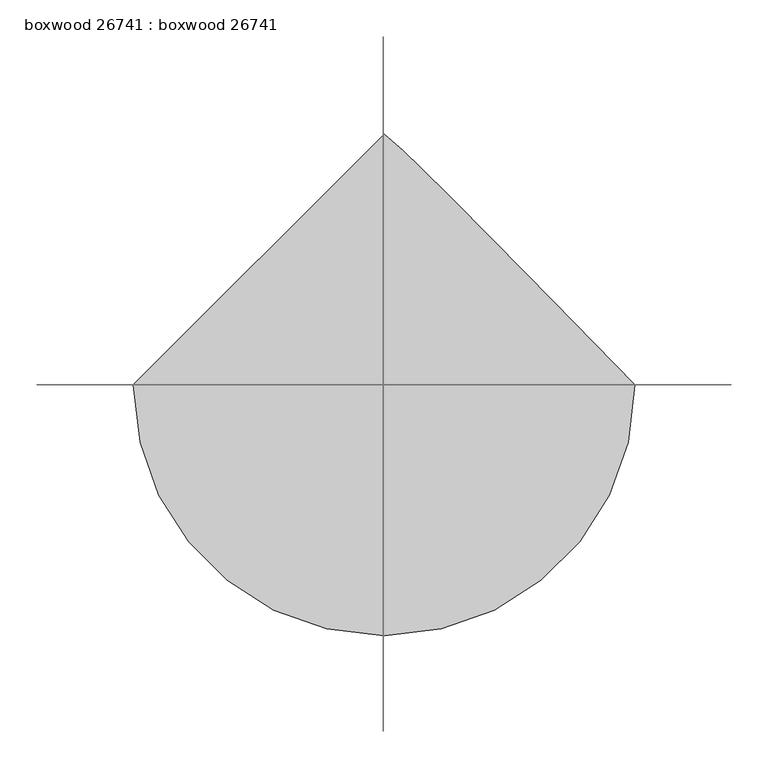
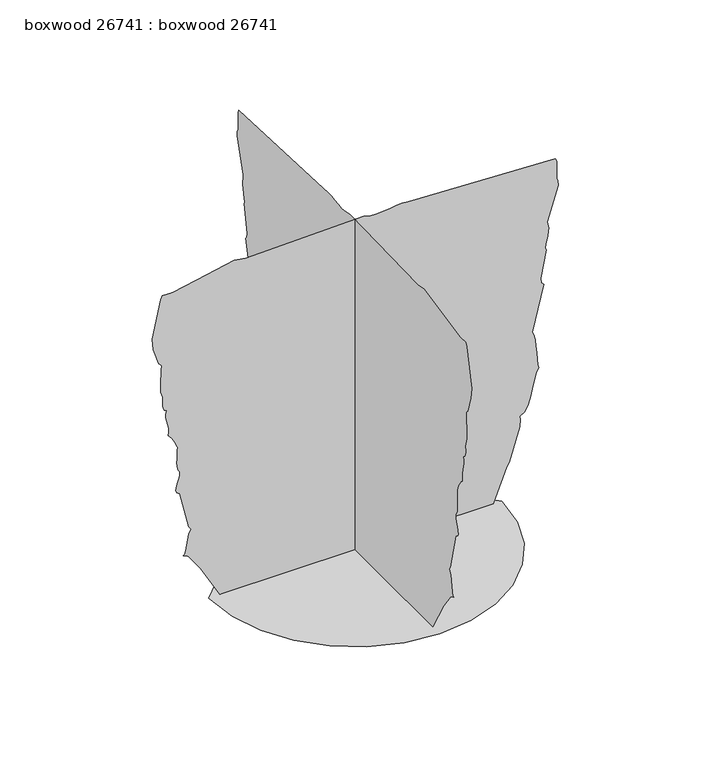
"""IFC4 building model written with IfcOpenShell, lengths in millimetres: proxy geometry, boxwood 26741 : boxwood 26741."""

import ifcopenshell
import ifcopenshell.guid

model = None  # the IFC model being written
_history = None  # IfcOwnerHistory: only IFC2X3 demands one
_inside = {}  # id of a spatial element -> (the spatial element, [elements in it])
_under = {}  # id of a project, library or spatial element -> (it, [spatial elements below it])
_declared = {}  # id of a project -> (the project, [libraries it declares])
_typed = {}  # id of a type object -> (the type object, [elements of that type])
_made_of = {}  # id of a material, layer set ... -> (it, [elements and type objects made of it])


def new_model(schema):
    """Start an empty IFC model of exactly this schema.

    Asked for "IFC4X3", IfcOpenShell would pick the latest addendum, in which some entities
    have other attributes; the version numbers below select the first issue.
    IFC2X3 requires an IfcOwnerHistory on every rooted entity: one is made here for all.
    """
    global model, _history
    if schema == "IFC4X3":
        model = ifcopenshell.file(schema_version=(4, 3, 0, 0))
    else:
        model = ifcopenshell.file(schema=schema)
    _inside.clear()
    _under.clear()
    _declared.clear()
    _typed.clear()
    _made_of.clear()
    _history = None
    if model.schema == "IFC2X3":
        org = make("IfcOrganization", Name="unknown")
        user = make(
            "IfcPersonAndOrganization",
            ThePerson=make("IfcPerson", FamilyName="unknown"),
            TheOrganization=org,
        )
        app = make(
            "IfcApplication",
            ApplicationDeveloper=org,
            Version="unknown",
            ApplicationFullName="unknown",
            ApplicationIdentifier="unknown",
        )
        _history = make(
            "IfcOwnerHistory",
            OwningUser=user,
            OwningApplication=app,
            ChangeAction="ADDED",
            CreationDate=0,
        )
    return model


def make(cls, **values):
    """One entity of the class cls with the attributes given. An attribute that is None is left unset."""
    return model.create_entity(
        cls, **{name: value for name, value in values.items() if value is not None}
    )


def rooted(cls, **values):
    """An entity with a GlobalId (a new one), such as an element, a storey or a relation."""
    return make(cls, GlobalId=ifcopenshell.guid.new(), OwnerHistory=_history, **values)


def si_unit(unit_type, name, prefix=None):
    """IfcSIUnit, for example si_unit("LENGTHUNIT", "METRE", prefix="MILLI")."""
    return make("IfcSIUnit", UnitType=unit_type, Prefix=prefix, Name=name)


def assignment(units):
    """IfcUnitAssignment: the units of a project."""
    return None if units is None else make("IfcUnitAssignment", Units=units)


def point(xyz):
    """IfcCartesianPoint."""
    return None if xyz is None else make("IfcCartesianPoint", Coordinates=xyz)


def direction(xyz):
    """IfcDirection."""
    return None if xyz is None else make("IfcDirection", DirectionRatios=xyz)


def frame(location, z_axis=None, x_axis=None):
    """IfcAxis2Placement3D, a coordinate frame: its origin and axes. An axis left out is left unset."""
    return make(
        "IfcAxis2Placement3D",
        Location=point(location),
        Axis=direction(z_axis),
        RefDirection=direction(x_axis),
    )


def origin():
    """The frame at (0, 0, 0) with its axes left unset."""
    return frame((0.0, 0.0, 0.0))


def place(relative_to, where):
    """IfcLocalPlacement: puts the frame where relative to a parent placement (None: the world)."""
    return make(
        "IfcLocalPlacement", PlacementRelTo=relative_to, RelativePlacement=where
    )


def context(
    kind, dimensions, precision=None, world=None, true_north=None, identifier=None
):
    """IfcGeometricRepresentationContext, for example the 3D "Model" context."""
    return make(
        "IfcGeometricRepresentationContext",
        ContextIdentifier=identifier,
        ContextType=kind,
        CoordinateSpaceDimension=dimensions,
        Precision=precision,
        WorldCoordinateSystem=world,
        TrueNorth=true_north,
    )


def project(units=None, contexts=None):
    """IfcProject with its units and contexts."""
    return rooted(
        "IfcProject",
        Name="project",
        RepresentationContexts=contexts,
        UnitsInContext=assignment(units),
    )


def spatial(cls, under=None, at=None, **own):
    """A site, building, storey or space (cls), placed at a placement, below another one or the project."""
    s = rooted(cls, ObjectPlacement=at, **own)
    if under is not None:
        _under.setdefault(under.id(), (under, []))[1].append(s)
    return s


def point_list(points):
    """IfcCartesianPointList2D or 3D."""
    cls = (
        "IfcCartesianPointList2D" if len(points[0]) == 2 else "IfcCartesianPointList3D"
    )
    return make(cls, CoordList=points)


def triangles(points, corners, closed=None, point_numbers=None):
    """IfcTriangulatedFaceSet: each triangle names its three corners, points numbered from 1."""
    return make(
        "IfcTriangulatedFaceSet",
        Coordinates=point_list(points),
        Closed=closed,
        CoordIndex=corners,
        PnIndex=point_numbers,
    )


def shape(context_of_items, identifier, shape_type, items):
    """IfcShapeRepresentation: the items that make up one representation, for example the "Body"."""
    return make(
        "IfcShapeRepresentation",
        ContextOfItems=context_of_items,
        RepresentationIdentifier=identifier,
        RepresentationType=shape_type,
        Items=items,
    )


def source(mapping_origin, context_of_items, identifier, shape_type, items):
    """IfcRepresentationMap: a shape defined once, which mapped items show again and again."""
    return make(
        "IfcRepresentationMap",
        MappingOrigin=mapping_origin,
        MappedRepresentation=shape(context_of_items, identifier, shape_type, items),
    )


def transform(
    local_origin,
    x_axis=None,
    y_axis=None,
    z_axis=None,
    scale=None,
    scale2=None,
    scale3=None,
    uniform=True,
):
    """IfcCartesianTransformationOperator3D, or its non-uniform kind. x_axis, y_axis, z_axis: its Axis1, 2, 3."""
    if uniform:
        return make(
            "IfcCartesianTransformationOperator3D",
            Axis1=direction(x_axis),
            Axis2=direction(y_axis),
            LocalOrigin=point(local_origin),
            Scale=scale,
            Axis3=direction(z_axis),
        )
    return make(
        "IfcCartesianTransformationOperator3DnonUniform",
        Axis1=direction(x_axis),
        Axis2=direction(y_axis),
        LocalOrigin=point(local_origin),
        Scale=scale,
        Axis3=direction(z_axis),
        Scale2=scale2,
        Scale3=scale3,
    )


def mapped(mapping_source, mapping_target):
    """IfcMappedItem: shows the shape of a source again, moved by a transform."""
    return make(
        "IfcMappedItem", MappingSource=mapping_source, MappingTarget=mapping_target
    )


def made_of(thing, what):
    """Note that an element or type object is made of a material, layer set ...; save() writes the relation."""
    if what is not None:
        _made_of.setdefault(what.id(), (what, []))[1].append(thing)
    return thing


def element(
    cls,
    number,
    at=None,
    inside=None,
    cuts=None,
    type_object=None,
    material=None,
    context=None,
    identifier="Body",
    shape_type=None,
    held_by="IfcProductDefinitionShape",
    body=None,
    shapes=None,
    **own,
):
    """One element of the class cls, such as IfcWall. Its Tag is "e" and its number.

    at: its placement. inside: the storey or other place that contains it. cuts: it is an
    opening in that element (IfcRelVoidsElement). A single representation is given by context,
    identifier, shape_type and body (its items); several are given by shapes. held_by: the class
    of the entity that holds the representations. save() writes the other relations.
    """
    e = rooted(cls, Tag="e%d" % number, ObjectPlacement=at, **own)
    if body is not None:
        shapes = [shape(context, identifier, shape_type, body)]
    if shapes is not None:
        e.Representation = make(held_by, Representations=shapes)
    if inside is not None:
        _inside.setdefault(inside.id(), (inside, []))[1].append(e)
    if cuts is not None:
        rooted(
            "IfcRelVoidsElement", RelatingBuildingElement=cuts, RelatedOpeningElement=e
        )
    if type_object is not None:
        _typed.setdefault(type_object.id(), (type_object, []))[1].append(e)
    return made_of(e, material)


def aggregate(whole, parts):
    """IfcRelAggregates: a whole, such as a stair, and the parts it consists of."""
    return rooted("IfcRelAggregates", RelatingObject=whole, RelatedObjects=parts)


def save(model, path):
    """Write the relations noted so far, then the file.

    IfcRelAggregates (storeys below a building ...), IfcRelContainedInSpatialStructure (elements
    in a storey), IfcRelDefinesByType, IfcRelAssociatesMaterial and IfcRelDeclares: one each for
    every whole, place, type object, material and project.
    """
    for whole, parts in _under.values():
        aggregate(whole, parts)
    for where, things in _inside.values():
        rooted(
            "IfcRelContainedInSpatialStructure",
            RelatedElements=things,
            RelatingStructure=where,
        )
    for kind, things in _typed.values():
        rooted("IfcRelDefinesByType", RelatedObjects=things, RelatingType=kind)
    for what, things in _made_of.values():
        rooted("IfcRelAssociatesMaterial", RelatedObjects=things, RelatingMaterial=what)
    for by, libraries in _declared.values():
        rooted("IfcRelDeclares", RelatingContext=by, RelatedDefinitions=libraries)
    model.write(path)


def boxwood_26741_boxwood_26741_9aa5a226(model_context):
    return source(origin(), model_context, "Body", "Tessellation", [
        triangles([(-340.161904, 0.0, 0.0), (-331.1677583, -77.9424445, 0.0), (-305.5569305, -149.5201522, 0.0), (-265.3792049, -212.6823306, 0.0), (-212.6823306, -265.3792049, 0.0), (-149.5201522, -305.5569305, 0.0), (-77.9424445, -331.1677583, 0.0), (1.49e-05, -340.161904, 0.0), (77.9424445, -331.1677583, 0.0), (149.5201522, -305.5569305, 0.0), (212.6823306, -265.3792049, 0.0), (265.3792049, -212.6823306, 0.0), (305.5569305, -149.5201522, 0.0), (331.1677583, -77.9424445, 0.0), (340.161904, 2.97e-05, 0.0), (229.6165077, 113.3919522, 0.0), (147.6639246, 196.877445, 0.0), (89.5385572, 255.4401858, 0.0), (50.4748806, 294.0659713, 0.0), (25.7075946, 317.7387815, 0.0), (10.4710485, 331.4420875, 0.0), (-4.46e-05, 340.161904, 0.0), (-314.391057, 3.72e-05, 1.1804295), (-359.6030502, 3.25e-05, 80.9365932), (-387.8072153, 3.02e-05, 119.3439327), (-399.7375917, 2.98e-05, 125.1409807), (-396.5295753, 2.97e-05, 127.6759005), (-393.8092472, 2.92e-05, 136.0634881), (-391.3784363, 2.85e-05, 147.9626255), (-389.0442038, 2.77e-05, 161.0321948), (-386.6159363, 2.7e-05, 172.9315956), (-383.8930647, 2.65e-05, 181.3191832), (-380.6875917, 2.64e-05, 183.8540939), (-386.4178379, 2.59e-05, 191.475867), (-407.8706709, 2.06e-05, 279.9816748), (-415.0715758, 2.03e-05, 285.8922515), (-417.4159822, 1.99e-05, 291.1246538), (-416.3669546, 1.95e-05, 298.5846272), (-413.3773842, 1.9e-05, 307.4187355), (-409.9052124, 1.84e-05, 316.7735787), (-407.3982433, 1.79e-05, 325.7905792), (-407.3144185, 1.74e-05, 333.6213876), (-411.0989985, 1.7e-05, 339.4049735), (-412.8821019, 1.68e-05, 343.3826014), (-413.8320439, 1.64e-05, 350.1263031), (-414.1444885, 1.59e-05, 358.7927799), (-414.0123745, 1.54e-05, 368.5362259), (-413.6237718, 1.48e-05, 378.5158856), (-413.1741989, 1.42e-05, 387.8859532), (-412.8516169, 1.37e-05, 395.8056733), (-413.5475773, 1.36e-05, 397.7894185), (-415.5668581, 1.33e-05, 402.5595489), (-418.5996308, 1.29e-05, 409.0720874), (-422.335958, 1.25e-05, 416.2857096), (-426.4660111, 1.21e-05, 423.1538587), (-430.6849397, 1.17e-05, 428.6300869), (-434.6803717, 1.15e-05, 431.6729971), (-433.0471501, 1.1e-05, 440.9821309), (-433.7685087, 1.04e-05, 450.5350362), (-435.8335353, 9.9e-06, 460.1032385), (-438.2363683, 9.3e-06, 469.4580454), (-439.9737259, 8.8e-06, 478.3709098), (-440.034696, 8.3e-06, 486.6106685), (-437.4134171, 7.8e-06, 493.9512815), (-443.2020899, 7.6e-06, 497.9797056), (-446.1205164, 7.3e-06, 503.1613297), (-447.0831757, 6.9e-06, 509.2624108), (-447.0095246, 6.6e-06, 516.0543654), (-446.8114263, 6.1e-06, 523.3111536), (-447.4083012, 5.6e-06, 530.7990686), (-449.7146284, 5.2e-06, 538.2920706), (-451.312278, 4.9e-06, 544.3448625), (-452.0082384, 4.4e-06, 552.960543), (-452.0184122, 3.7e-06, 563.4380648), (-451.5713828, 3e-06, 575.0738008), (-450.8830164, 2.3e-06, 587.161653), (-450.1769185, 1.6e-06, 599.0006106), (-449.6740059, 1e-06, 609.884503), (-455.9351063, 5e-07, 616.20403), (-468.9576762, -1.9e-06, 655.9295849), (-471.3528789, -3.4e-06, 681.38806), (-452.1758881, -8.8e-06, 772.6680262), (-448.2312887, -9.3e-06, 780.8340975), (-424.9242448, -9.2e-06, 779.2695127), (-369.5370006, -9.9e-06, 791.4970367), (-280.9036933, -1.1e-05, 809.3710184), (-254.2463815, -1.07e-05, 804.8396816), (19.1367407, -1.11e-05, 811.6748022), (35.370009, -1.09e-05, 807.659059), (50.7118619, -1.08e-05, 806.6938562), (65.4184633, -1.09e-05, 807.7555647), (79.7468584, -1.1e-05, 809.8129972), (93.9523139, -1.11e-05, 811.837365), (108.2921454, -1.11e-05, 812.8000242), (123.0221057, -1.11e-05, 811.6748022), (464.7514286, -1.02e-05, 797.3212452), (467.4463586, -9.9e-06, 790.6791361), (467.5250965, -7.3e-06, 748.7767519), (470.2200628, -6.9e-06, 742.132172), (471.0074421, -6.3e-06, 730.722476), (446.1992907, -1.4e-06, 649.650753), (447.5784943, -8e-07, 638.6728621), (448.9932698, -4e-07, 632.8486536), (448.3227076, 0.0, 624.6114384), (446.3999325, 6e-07, 614.9264191), (444.0605767, 1.2e-06, 604.756255), (442.1378016, 1.8e-06, 595.0686922), (441.4672394, 2.3e-06, 586.8314406), (442.8795078, 2.7e-06, 581.0072322), (430.5681227, 6.5e-06, 516.2728114), (432.2445102, 7.2e-06, 504.59896), (437.7537669, 7.6e-06, 498.820461), (410.7154827, 1.41e-05, 389.8950966), (414.6016554, 1.45e-05, 382.811045), (417.3397877, 1.52e-05, 370.1135642), (419.2981347, 1.62e-05, 353.9591723), (420.8348505, 1.72e-05, 336.5119088), (422.3156467, 1.82e-05, 319.9231685), (424.1038007, 1.9e-05, 306.3570271), (426.5625169, 1.95e-05, 297.9699481), (420.4843268, 2.02e-05, 287.3705225), (415.6710305, 2.11e-05, 270.9595874), (411.3047636, 2.23e-05, 251.374918), (406.5625749, 2.35e-05, 231.2497293), (400.6266, 2.46e-05, 213.2215782), (392.6738514, 2.54e-05, 199.9259508), (381.8813779, 2.58e-05, 193.9993685), (383.6035111, 2.63e-05, 184.6265031), (381.7493002, 2.73e-05, 168.2889829), (357.4541988, 3.19e-05, 89.6124717), (351.8814649, 3.25e-05, 80.6919951), (319.8571115, 3.72e-05, 1.0471049), (-1.3669569, -313.0245343, 1.1804269), (-1.3669569, -358.2365275, 80.9365932), (-1.3669569, -386.4381492, 119.3439327), (-1.3669569, -398.371069, 125.1409807), (-1.3669569, -395.1630527, 127.6759005), (-1.3669569, -392.4427245, 136.0634881), (-1.3669569, -390.0119136, 147.9626255), (-1.3669569, -387.6776811, 161.0324491), (-1.3669569, -385.2469065, 172.9315956), (-1.3669569, -382.526542, 181.3191832), (-1.3669569, -379.3185256, 183.8540939), (-1.3669569, -385.0513152, 191.475867), (-1.3669569, -406.5041482, 279.9816748), (-1.3669569, -413.7050531, 285.8922515), (-1.3669569, -416.046916, 291.1246538), (-1.3669569, -414.9979248, 298.5846272), (-1.3669569, -412.0108615, 307.4187355), (-1.3669569, -408.5386897, 316.7735787), (-1.3669569, -406.0317206, 325.7905792), (-1.3669569, -405.9453524, 333.6213876), (-1.3669569, -409.7324759, 339.4049735), (-1.3669569, -411.5130358, 343.3826014), (-1.3669569, -412.4655212, 350.1263031), (-1.3669569, -412.7779658, 358.7927799), (-1.3669569, -412.6458881, 368.5362259), (-1.3669569, -412.2572491, 378.5158856), (-1.3669569, -411.8076762, 387.8859532), (-1.3669569, -411.4850942, 395.8056733), (-1.3669569, -412.1810546, 397.7894185), (-1.3669569, -414.2003354, 402.5595489), (-1.3669569, -417.2331081, 409.0720874), (-1.3669569, -420.9669282, 416.2857096), (-1.3669569, -425.0994884, 423.1538587), (-1.3669569, -429.318417, 428.6300869), (-1.3669569, -433.3113055, 431.6729971), (-1.3669569, -431.6806274, 440.9821309), (-1.3669569, -432.401986, 450.5350362), (-1.3669569, -434.4670126, 460.1032385), (-1.3669569, -436.8698456, 469.4580454), (-1.3669569, -438.6046597, 478.3709098), (-1.3669569, -438.6681733, 486.6132119), (-1.3669569, -436.0468944, 493.9512815), (-1.3669569, -441.8355672, 497.9797056), (-1.3669569, -444.75403, 503.1613297), (-1.3669569, -445.7166893, 509.2624108), (-1.3669569, -445.6430019, 516.0543654), (-1.3669569, -445.4449036, 523.3111536), (-1.3669569, -446.0417785, 530.7990686), (-1.3669569, -448.3481057, 538.2920706), (-1.3669569, -449.9457553, 544.3448625), (-1.3669569, -450.6392086, 552.960543), (-1.3669569, -450.6518895, 563.4380648), (-1.3669569, -450.2023167, 575.0738008), (-1.3669569, -449.5139866, 587.161653), (-1.3669569, -448.8078524, 599.0006106), (-1.3669569, -448.3049397, 609.884503), (-1.3669569, -454.5685836, 616.20403), (-1.3669569, -467.5911535, 655.9295849), (-1.3669569, -469.9863562, 681.38806), (-1.3669569, -450.8093654, 772.6680262), (-1.3669569, -446.864766, 780.8340975), (-1.3669569, -423.5577221, 779.2695127), (-1.3669569, -368.1704779, 791.4970367), (-1.3669569, -279.5371706, 809.3710184), (-1.3669569, -252.8793683, 804.8396816), (-1.3669569, 20.5037698, 811.6748022), (-1.3669569, 36.7367838, 807.659059), (-1.3669569, 52.0788933, 806.6938562), (-1.3669569, 66.7854902, 807.7555647), (-1.3669569, 81.1138897, 809.8129972), (-1.3669569, 95.3193453, 811.837365), (-1.3669569, 109.6591677, 812.8000242), (-1.3669569, 124.3891371, 811.6748022), (-1.3669569, 466.1179513, 797.3212452), (-1.3669569, 468.8128813, 790.6791361), (-1.3669569, 468.8916192, 748.7767519), (-1.3669569, 471.5865855, 742.132172), (-1.3669569, 472.3739648, 730.722476), (-1.3669569, 447.565777, 649.650753), (-1.3669569, 448.9475604, 638.6754055), (-1.3669569, 450.3597925, 632.8486536), (-1.3669569, 449.6892303, 624.6114384), (-1.3669569, 447.7664552, 614.9264191), (-1.3669569, 445.4270994, 604.756255), (-1.3669569, 443.5068678, 595.0686922), (-1.3669569, 442.8337621, 586.8314406), (-1.3669569, 444.2485376, 581.0072322), (-1.3669569, 431.9371888, 516.2728114), (-1.3669569, 433.6135763, 504.59896), (-1.3669569, 439.1228331, 498.820461), (-1.3669569, 412.0820054, 389.8950966), (-1.3669569, 415.9681781, 382.811045), (-1.3669569, 418.7088538, 370.1135642), (-1.3669569, 420.6646574, 353.9591723), (-1.3669569, 422.2013369, 336.5119088), (-1.3669569, 423.6821694, 319.9231685), (-1.3669569, 425.4703234, 306.3570271), (-1.3669569, 427.9290396, 297.9699481), (-1.3669569, 421.8508495, 287.3705225), (-1.3669569, 417.0375169, 270.9595874), (-1.3669569, 412.6712863, 251.374918), (-1.3669569, 407.9290976, 231.2497293), (-1.3669569, 401.9931227, 213.2215782), (-1.3669569, 394.0403741, 199.9259508), (-1.3669569, 383.2479006, 193.9993685), (-1.3669569, 384.9700338, 184.6265031), (-1.3669569, 383.1158229, 168.2892373), (-1.3669569, 358.8207215, 89.6124717), (-1.3669569, 353.2479876, 80.6919951), (-1.3669569, 321.2261776, 1.0470998)], [[21, 22, 1], [20, 21, 1], [19, 20, 1], [18, 19, 1], [17, 18, 1], [17, 1, 2], [17, 2, 3], [17, 3, 4], [16, 17, 4], [16, 4, 5], [16, 5, 6], [16, 6, 7], [16, 7, 8], [16, 8, 9], [16, 9, 10], [16, 10, 11], [16, 11, 12], [15, 16, 12], [14, 15, 12], [13, 14, 12], [25, 26, 27], [131, 132, 23], [82, 83, 84], [95, 96, 97], [95, 97, 98], [25, 27, 28], [56, 57, 58], [131, 23, 24], [130, 131, 24], [129, 130, 24], [128, 129, 24], [127, 128, 24], [95, 98, 99], [95, 99, 100], [95, 100, 101], [95, 101, 102], [127, 24, 25], [127, 25, 28], [127, 28, 29], [127, 29, 30], [127, 30, 31], [127, 31, 32], [127, 32, 33], [127, 33, 34], [127, 34, 35], [111, 112, 113], [95, 102, 103], [95, 103, 104], [95, 104, 105], [95, 105, 106], [95, 106, 107], [95, 107, 108], [119, 120, 121], [81, 82, 84], [95, 108, 109], [95, 109, 110], [94, 95, 110], [93, 94, 110], [92, 93, 110], [91, 92, 110], [91, 110, 111], [90, 91, 111], [90, 111, 113], [89, 90, 113], [126, 127, 35], [125, 126, 35], [124, 125, 35], [123, 124, 35], [122, 123, 35], [121, 122, 35], [119, 121, 35], [118, 119, 35], [117, 118, 35], [116, 117, 35], [115, 116, 35], [114, 115, 35], [113, 114, 35], [89, 113, 35], [88, 89, 35], [87, 88, 35], [87, 35, 36], [87, 36, 37], [81, 84, 85], [80, 81, 85], [79, 80, 85], [78, 79, 85], [78, 85, 86], [78, 86, 87], [77, 78, 87], [76, 77, 87], [75, 76, 87], [74, 75, 87], [73, 74, 87], [72, 73, 87], [71, 72, 87], [70, 71, 87], [69, 70, 87], [68, 69, 87], [67, 68, 87], [66, 67, 87], [65, 66, 87], [64, 65, 87], [55, 56, 58], [62, 63, 64], [62, 64, 87], [61, 62, 87], [60, 61, 87], [59, 60, 87], [58, 59, 87], [55, 58, 87], [54, 55, 87], [53, 54, 87], [52, 53, 87], [51, 52, 87], [50, 51, 87], [49, 50, 87], [48, 49, 87], [47, 48, 87], [46, 47, 87], [45, 46, 87], [44, 45, 87], [43, 44, 87], [42, 43, 87], [41, 42, 87], [37, 38, 39], [37, 39, 40], [87, 37, 40], [41, 87, 40], [135, 136, 137], [241, 242, 133], [192, 193, 194], [205, 206, 207], [205, 207, 208], [135, 137, 138], [166, 167, 168], [241, 133, 134], [240, 241, 134], [239, 240, 134], [238, 239, 134], [237, 238, 134], [205, 208, 209], [205, 209, 210], [205, 210, 211], [205, 211, 212], [237, 134, 135], [237, 135, 138], [237, 138, 139], [237, 139, 140], [237, 140, 141], [237, 141, 142], [237, 142, 143], [237, 143, 144], [237, 144, 145], [221, 222, 223], [205, 212, 213], [205, 213, 214], [205, 214, 215], [205, 215, 216], [205, 216, 217], [205, 217, 218], [229, 230, 231], [191, 192, 194], [205, 218, 219], [205, 219, 220], [204, 205, 220], [203, 204, 220], [202, 203, 220], [201, 202, 220], [201, 220, 221], [200, 201, 221], [200, 221, 223], [199, 200, 223], [236, 237, 145], [235, 236, 145], [234, 235, 145], [233, 234, 145], [232, 233, 145], [231, 232, 145], [229, 231, 145], [228, 229, 145], [227, 228, 145], [226, 227, 145], [225, 226, 145], [224, 225, 145], [223, 224, 145], [199, 223, 145], [198, 199, 145], [197, 198, 145], [197, 145, 146], [197, 146, 147], [191, 194, 195], [190, 191, 195], [189, 190, 195], [188, 189, 195], [188, 195, 196], [188, 196, 197], [187, 188, 197], [186, 187, 197], [185, 186, 197], [184, 185, 197], [183, 184, 197], [182, 183, 197], [181, 182, 197], [180, 181, 197], [179, 180, 197], [178, 179, 197], [177, 178, 197], [176, 177, 197], [175, 176, 197], [174, 175, 197], [165, 166, 168], [172, 173, 174], [172, 174, 197], [171, 172, 197], [170, 171, 197], [169, 170, 197], [168, 169, 197], [165, 168, 197], [164, 165, 197], [163, 164, 197], [162, 163, 197], [161, 162, 197], [160, 161, 197], [159, 160, 197], [158, 159, 197], [157, 158, 197], [156, 157, 197], [155, 156, 197], [154, 155, 197], [153, 154, 197], [152, 153, 197], [151, 152, 197], [147, 148, 149], [147, 149, 150], [197, 147, 150], [151, 197, 150]], closed=False),
    ])


if __name__ == "__main__":
    model = new_model("IFC4")
    model_context = context("Model", 3, world=origin())
    ifc_project = project(units=[si_unit("LENGTHUNIT", "METRE", prefix="MILLI")], contexts=[model_context])
    site = spatial("IfcSite", under=ifc_project)
    building = spatial("IfcBuilding", under=site)
    placement = place(None, origin())
    boxwood_26741_boxwood_26741_shape = boxwood_26741_boxwood_26741_9aa5a226(model_context)
    element("IfcBuildingElementProxy", 1, Name="boxwood 26741 : boxwood 26741", ObjectType="boxwood 26741 : boxwood 26741", at=placement, inside=building, context=model_context, shape_type="MappedRepresentation", body=[
        mapped(boxwood_26741_boxwood_26741_shape, transform((0.0, 0.0, 0.0), x_axis=(1.0, 0.0, 0.0), y_axis=(0.0, 1.0, 0.0), z_axis=(0.0, 0.0, 1.0))),
    ])
    save(model, "model.ifc")

# Revit data of these elements
# Type "boxwood 26741 : boxwood 26741"
#   built-in parameter 1005195 = "RPC-16-G0M3-8AG0-UBW3-U000-ST1L-LVER-AU"
#   Height = 0
